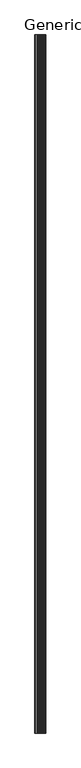
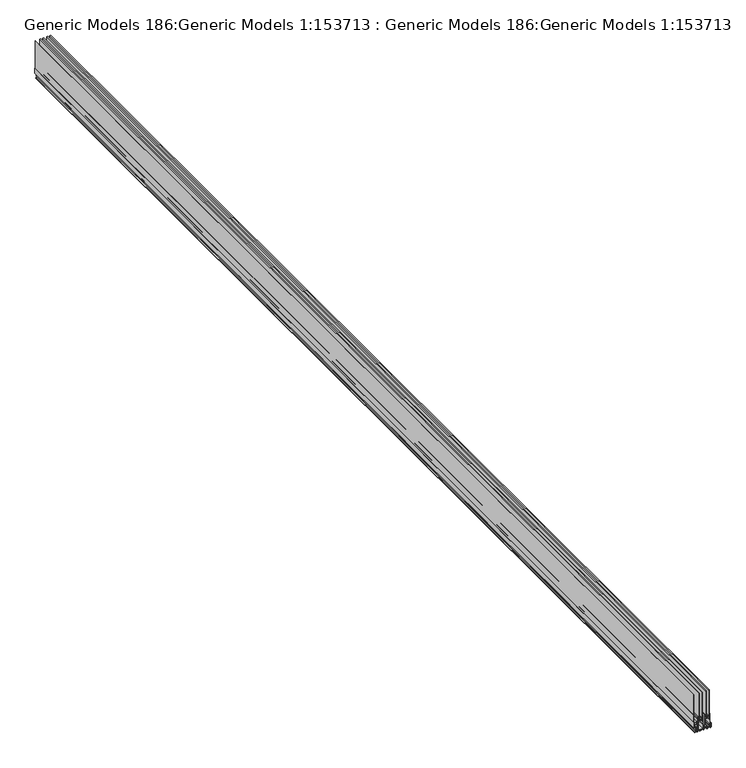
"""IFC4 building model written with IfcOpenShell, lengths in millimetres: proxy geometry, Generic Models 186:Generic Models 1:153713 : Generic Models 186:Generic Models 1:153713."""

from ifc_helpers import new_model, si_unit, frame, origin, place, context, project, spatial, polyline, outline, extrude, source, transform, mapped, element, save


def generic_models_186_generic_models_1_153713_generic_models_36636e81(model_context):
    return source(origin(), model_context, "Body", "SweptSolid", [
        extrude(outline(polyline([(-5328.1713019, -273.9974793), (-5328.1713019, 7612.7025207), (-5313.8414704, 7612.7025207), (-5313.8414704, -273.9974793), (-5328.1713019, -273.9974793)])), frame((0.0, 0.0, 3559.9182556), z_axis=(0.0, 0.0, 1.0), x_axis=(1.0, 0.0, 0.0)), (0.0, 0.0, 1.0), 7.9798298),
        extrude(outline(polyline([(-5313.0477204, -273.9974793), (-5313.0477204, 7612.7025207), (-5308.3063862, 7612.7025207), (-5308.3063862, -273.9974793), (-5313.0477204, -273.9974793)])), frame((0.0, 0.0, 3559.1245056), z_axis=(0.0, 0.0, 1.0), x_axis=(1.0, 0.0, 0.0)), (0.0, 0.0, 1.0), 191.9290887),
        extrude(outline(polyline([(-5333.7063862, -273.9974793), (-5333.7063862, 7612.7025207), (-5328.9650519, 7612.7025207), (-5328.9650519, -273.9974793), (-5333.7063862, -273.9974793)])), frame((0.0, 0.0, 3559.1245056), z_axis=(0.0, 0.0, 1.0), x_axis=(1.0, 0.0, 0.0)), (0.0, 0.0, 1.0), 191.9290887),
        extrude(outline(polyline([(-5279.8266395, -273.9974793), (-5279.8266395, 7612.7025207), (-5265.496808, 7612.7025207), (-5265.496808, -273.9974793), (-5279.8266395, -273.9974793)])), frame((0.0, 0.0, 3559.9182556), z_axis=(0.0, 0.0, 1.0), x_axis=(1.0, 0.0, 0.0)), (0.0, 0.0, 1.0), 7.9798298),
        extrude(outline(polyline([(3489.5285151, -5346.1523792), (3489.5285151, -5344.8823766), (3542.3605081, -5344.8823766), (3542.3605081, -5347.9303852), (3548.5411748, -5347.9303852), (3548.5411748, -5366.2924677), (3751.0535943, -5366.2924677), (3751.0535943, -5367.0862177), (3548.5411748, -5367.0862177), (3548.5411748, -5368.6737177), (3512.2023941, -5368.6737177), (3509.6360367, -5358.5983817), (3489.5285048, -5358.5983817), (3489.5285048, -5357.3283792), (3502.4825048, -5357.3283792), (3502.4825048, -5346.1523792), (3489.5285151, -5346.1523792)]), holes=[polyline([(3533.0471765, -5356.3970561), (3531.3538406, -5356.3970561), (3531.3538406, -5346.2370561), (3503.7525039, -5346.2370561), (3503.7525039, -5357.3283905), (3510.6532105, -5357.3283905), (3513.1287718, -5367.3190484), (3516.8758337, -5367.3190484), (3516.8758337, -5364.9483922), (3518.1458354, -5364.9483922), (3518.1458354, -5367.3190622), (3541.0905056, -5367.3190622), (3541.0905056, -5360.1223955), (3547.2711748, -5360.1223955), (3547.2711748, -5349.2003766), (3541.0905081, -5349.2003766), (3541.0905081, -5346.1523955), (3533.0471765, -5346.1523955), (3533.0471765, -5356.3970561)])]), frame((0.0, -273.9974793, 0.0), z_axis=(0.0, 1.0, 0.0), x_axis=(0.0, 0.0, 1.0)), (0.0, 0.0, 1.0), 7886.7),
        extrude(outline(polyline([(-5264.703058, -273.9974793), (-5264.703058, 7612.7025207), (-5259.9617238, 7612.7025207), (-5259.9617238, -273.9974793), (-5264.703058, -273.9974793)])), frame((0.0, 0.0, 3559.1245056), z_axis=(0.0, 0.0, 1.0), x_axis=(1.0, 0.0, 0.0)), (0.0, 0.0, 1.0), 191.9290887),
        extrude(outline(polyline([(-5285.3617238, -273.9974793), (-5285.3617238, 7612.7025207), (-5280.6203895, 7612.7025207), (-5280.6203895, -273.9974793), (-5285.3617238, -273.9974793)])), frame((0.0, 0.0, 3559.1245056), z_axis=(0.0, 0.0, 1.0), x_axis=(1.0, 0.0, 0.0)), (0.0, 0.0, 1.0), 191.9290887),
        extrude(outline(polyline([(3504.7685151, -5252.0030441), (3496.1325048, -5252.0030441), (3496.1325048, -5250.2250502), (3489.4010387, -5250.2250502), (3487.9198372, -5267.0737169), (3484.4485039, -5267.0737169), (3484.4485039, -5266.0577246), (3481.1465117, -5266.0577246), (3481.1465117, -5268.767058), (3482.077845, -5269.6137246), (3482.7021637, -5270.6038543), (3483.0897685, -5271.5949246), (3483.2308992, -5272.5855246), (3483.1157956, -5273.5742432), (3482.7346976, -5274.5596691), (3482.077845, -5275.5403913), (3481.1465117, -5276.4717246), (3481.1465117, -5279.1810502), (3484.4485021, -5279.1810502), (3484.4485021, -5278.1650502), (3486.9038354, -5278.1650502), (3486.9038354, -5281.5517169), (3484.4485021, -5281.5517169), (3484.4485021, -5303.5650502), (3481.9085021, -5303.5650502), (3481.9085021, -5306.4437169), (3484.3638354, -5306.4437169), (3484.3638354, -5335.5690502), (3481.9085021, -5335.5690502), (3481.9085021, -5338.4477169), (3484.3638354, -5338.4477169), (3484.3638354, -5340.9030502), (3476.9978354, -5340.9030502), (3476.9978354, -5350.6397169), (3480.9771687, -5350.6397169), (3480.9771687, -5352.5870502), (3476.9978354, -5352.5870502), (3476.9978354, -5362.0697169), (3473.0185021, -5362.0697169), (3473.0185021, -5355.7197169), (3474.6271687, -5355.7197169), (3474.6271687, -5342.9350502), (3473.0185021, -5342.9350502), (3473.0185021, -5338.4477169), (3479.5378354, -5338.4477169), (3479.5378354, -5334.7223835), (3481.9085021, -5333.1060199), (3481.9085021, -5325.5783905), (3473.0184995, -5325.5783905), (3473.0184995, -5323.1230571), (3474.9658329, -5323.1230571), (3476.7438329, -5322.1070571), (3477.3364952, -5322.6997195), (3478.4020598, -5323.0378724), (3479.6068593, -5322.9266454), (3480.3547069, -5322.278893), (3480.6628169, -5321.3259438), (3480.5484039, -5320.2991262), (3480.0286823, -5319.4297688), (3479.1208666, -5318.9492), (3478.3085492, -5318.9590508), (3477.336497, -5319.3130511), (3476.7438303, -5319.9057177), (3474.6271637, -5318.7203844), (3475.3891637, -5317.7043844), (3476.240338, -5317.0562532), (3477.1448995, -5316.630372), (3478.0868553, -5316.4248594), (3479.050213, -5316.4378338), (3480.01898, -5316.6674137), (3480.9771637, -5317.1117177), (3481.908497, -5317.8737177), (3481.908497, -5308.8990511), (3479.5378303, -5307.2166425), (3479.5378303, -5300.3477177), (3473.018497, -5300.3477177), (3473.018497, -5297.9770511), (3481.146497, -5297.9770511), (3481.146497, -5281.5517177), (3478.7758303, -5279.8693091), (3478.7758303, -5277.2337177), (3473.018497, -5277.2337177), (3473.018497, -5274.8630511), (3474.7118303, -5274.8630511), (3476.7438303, -5273.6777177), (3477.336497, -5274.3550588), (3478.3583227, -5274.6779926), (3479.5477736, -5274.5569292), (3480.3227217, -5273.9097749), (3480.6802895, -5272.9620539), (3480.6175998, -5271.9392905), (3480.1317752, -5271.0670089), (3479.2199383, -5270.5707332), (3478.3739527, -5270.560145), (3477.336497, -5270.8837255), (3476.7438303, -5271.5610588), (3474.6271637, -5270.2910588), (3475.3891637, -5269.3597255), (3476.4051637, -5268.5977255), (3477.5058303, -5268.1743922), (3478.7758303, -5268.0050588), (3478.7758303, -5263.6870502), (3485.8545301, -5263.6870502), (3486.9579804, -5250.2250441), (3477.8445151, -5250.2250441), (3477.8445151, -5252.5957108), (3475.3891817, -5252.5957108), (3475.3891817, -5254.2043775), (3473.0185151, -5254.2043775), (3473.0185151, -5250.2250441), (3475.3891817, -5250.2250441), (3475.3891817, -5247.7697108), (3504.7685151, -5247.7697108), (3504.7685151, -5252.0030441)])), frame((0.0, -273.9974793, 0.0), z_axis=(0.0, 1.0, 0.0), x_axis=(0.0, 0.0, 1.0)), (0.0, 0.0, 1.0), 7886.7),
        extrude(outline(polyline([(3490.8831748, -5288.6637142), (3493.2538415, -5286.4623809), (3493.2538415, -5282.5677117), (3500.1965108, -5282.5677117), (3500.1965108, -5287.4783905), (3537.1111775, -5287.4783905), (3537.1111775, -5284.2610571), (3538.7198442, -5284.2610571), (3538.7198442, -5287.4783792), (3553.6211687, -5287.4783792), (3554.4678354, -5287.3090458), (3555.3145021, -5286.8010458), (3555.8225021, -5285.9543792), (3555.9918354, -5285.1077125), (3555.9918354, -5278.7577125), (3555.8225056, -5277.9957125), (3554.5622266, -5276.7846656), (3553.5893497, -5276.6496403), (3552.6446253, -5277.0524864), (3551.8431723, -5277.9957125), (3551.6738389, -5278.7577125), (3551.6738389, -5281.3823792), (3549.8111723, -5281.3823792), (3549.8111723, -5274.9477125), (3551.9278389, -5273.7623792), (3552.4358389, -5274.3550571), (3553.7027031, -5274.795951), (3554.5125532, -5274.6805999), (3555.2139741, -5274.2264428), (3555.7378389, -5273.4237238), (3555.9071723, -5272.6617238), (3555.7378501, -5271.8997255), (3554.8811488, -5270.8269675), (3554.1168725, -5270.5434329), (3553.2787306, -5270.5938264), (3552.4358501, -5270.9683922), (3551.9278501, -5271.5610588), (3549.8111834, -5270.3757091), (3549.8111834, -5263.9410425), (3551.6738501, -5263.9410425), (3551.6738501, -5266.5657091), (3551.8431687, -5267.3277134), (3553.10627, -5268.5400146), (3554.0794605, -5268.6737856), (3555.0232441, -5268.2693135), (3555.8225021, -5267.3277134), (3555.9918458, -5266.5657134), (3555.9918458, -5260.2157238), (3555.8225125, -5259.2843905), (3555.3145125, -5258.5223905), (3554.4678458, -5258.0143905), (3553.6211792, -5257.8450571), (3538.7198458, -5257.8450571), (3538.7198458, -5261.0623905), (3537.1111792, -5261.0623905), (3537.1111792, -5257.8450571), (3500.1965117, -5257.8450571), (3500.1965117, -5262.7557228), (3494.6085117, -5262.7557228), (3494.6085117, -5255.4743878), (3579.7831775, -5255.4743878), (3579.7831775, -5257.8450467), (3560.73318, -5257.8450467), (3559.8018467, -5258.01438), (3559.0398467, -5258.52238), (3558.5318467, -5259.28438), (3558.3625031, -5260.2157134), (3558.3625031, -5285.1077238), (3558.5318364, -5285.9543905), (3559.0398364, -5286.8010571), (3559.8018364, -5287.3090571), (3560.7331697, -5287.4783905), (3579.7831697, -5287.4783905), (3579.7831697, -5289.8490571), (3492.0201162, -5289.8490571), (3489.0205081, -5292.4737142), (3487.0731748, -5294.5057142), (3485.4645081, -5296.7070475), (3486.9038415, -5293.7437142), (3488.7665081, -5291.1190475), (3490.8831748, -5288.6637142)])), frame((0.0, -273.9974793, 0.0), z_axis=(0.0, 1.0, 0.0), x_axis=(0.0, 0.0, 1.0)), (0.0, 0.0, 1.0), 7886.7),
        extrude(outline(polyline([(3537.1111792, -5306.189716), (3482.7551775, -5306.189716), (3482.7551775, -5303.8190502), (3579.7831775, -5303.8190502), (3579.7831775, -5306.1897091), (3560.73318, -5306.1897091), (3559.8018467, -5306.3590425), (3559.0398467, -5306.8670425), (3558.5318467, -5307.6290425), (3558.3625031, -5308.5603758), (3558.3625031, -5333.4523862), (3558.5318364, -5334.2990529), (3559.0398364, -5335.1457196), (3559.8018364, -5335.6537196), (3560.7331697, -5335.8230529), (3579.7831775, -5335.8230529), (3579.7831775, -5338.193715), (3482.7551775, -5338.193715), (3482.7551775, -5335.8230614), (3537.1111775, -5335.8230614), (3537.1111775, -5332.6057196), (3538.7198442, -5332.6057196), (3538.7198442, -5335.8230416), (3553.6211687, -5335.8230416), (3554.4678354, -5335.6537083), (3555.3145021, -5335.1457083), (3555.8225021, -5334.2990416), (3555.9918354, -5333.4523749), (3555.9918354, -5327.1023749), (3555.8225056, -5326.3403749), (3554.5622266, -5325.129328), (3553.5893497, -5324.9943027), (3552.6446253, -5325.3971488), (3551.8431723, -5326.3403749), (3551.6738389, -5327.1023749), (3551.6738389, -5329.7270416), (3549.8111723, -5329.7270416), (3549.8111723, -5323.2923749), (3551.9278389, -5322.1070416), (3552.4358389, -5322.6997196), (3553.7027031, -5323.1406134), (3554.5125532, -5323.0252623), (3555.2139741, -5322.5711052), (3555.7378389, -5321.7683862), (3555.9071723, -5321.0063862), (3555.7378501, -5320.2443879), (3554.8811488, -5319.1716299), (3554.1168725, -5318.8880953), (3553.2787306, -5318.9384888), (3552.4358501, -5319.3130546), (3551.9278501, -5319.9057213), (3549.8111834, -5318.7203716), (3549.8111834, -5312.2857049), (3551.6738501, -5312.2857049), (3551.6738501, -5314.9103716), (3551.8431687, -5315.6723758), (3553.10627, -5316.884677), (3554.0794605, -5317.018448), (3555.0232441, -5316.613976), (3555.8225021, -5315.6723758), (3555.9918458, -5314.9103758), (3555.9918458, -5308.5603862), (3555.8225125, -5307.6290529), (3555.3145125, -5306.8670529), (3554.4678458, -5306.3590529), (3553.6211792, -5306.1897196), (3538.7198458, -5306.1897196), (3538.7198458, -5309.4070529), (3537.1111792, -5309.4070529), (3537.1111792, -5306.189716)])), frame((0.0, -273.9974793, 0.0), z_axis=(0.0, 1.0, 0.0), x_axis=(0.0, 0.0, 1.0)), (0.0, 0.0, 1.0), 7886.7),
    ])


if __name__ == "__main__":
    model = new_model("IFC4")
    model_context = context("Model", 3, world=origin())
    ifc_project = project(units=[si_unit("LENGTHUNIT", "METRE", prefix="MILLI")], contexts=[model_context])
    site = spatial("IfcSite", under=ifc_project)
    building = spatial("IfcBuilding", under=site)
    placement = place(None, origin())
    generic_models_186_generic_models_1_153713_generic_models_shape = generic_models_186_generic_models_1_153713_generic_models_36636e81(model_context)
    element("IfcBuildingElementProxy", 1, Name="Generic Models 186:Generic Models 1:153713 : Generic Models 186:Generic Models 1:153713", ObjectType="Generic Models 186:Generic Models 1:153713 : Generic Models 186:Generic Models 1:153713", at=placement, inside=building, context=model_context, shape_type="MappedRepresentation", body=[
        mapped(generic_models_186_generic_models_1_153713_generic_models_shape, transform((0.0, 0.0, 0.0), x_axis=(1.0, 0.0, 0.0), y_axis=(0.0, 1.0, 0.0), z_axis=(0.0, 0.0, 1.0))),
    ])
    save(model, "model.ifc")

# Revit data of these elements
# Type "Generic Models 186:Generic Models 1:153713 : Generic Models 186:Generic Models 1:153713"
#   NameOverride = "Generic Models 186:Generic Models 1:153713"
#   ObjectTypeOverride = "Generic Models 186:Generic Models 1"
#   Reference = "Generic Models 1"
#   Category = "Generic Models"
#   Tag = "153713"
# Element 1 (IfcBuildingElementProxy, "Generic Models 186:Generic Models 1:153713 : Generic Models 186:Generic Models 1:153713")
#   Materials on its faces: "_SIDING DOOR PER SCHEDULE 11160"
# Materials
#   "_SIDING DOOR PER SCHEDULE 11160": class "Unassigned", colour RGB 255 255 255, transparency 0
